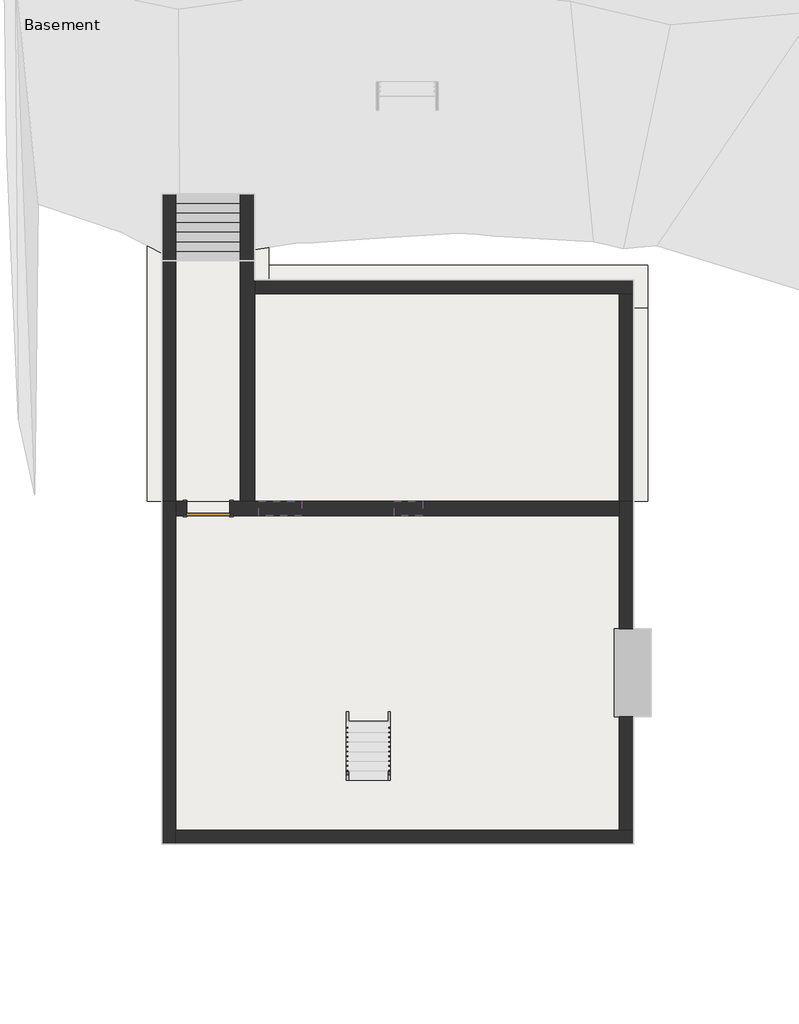
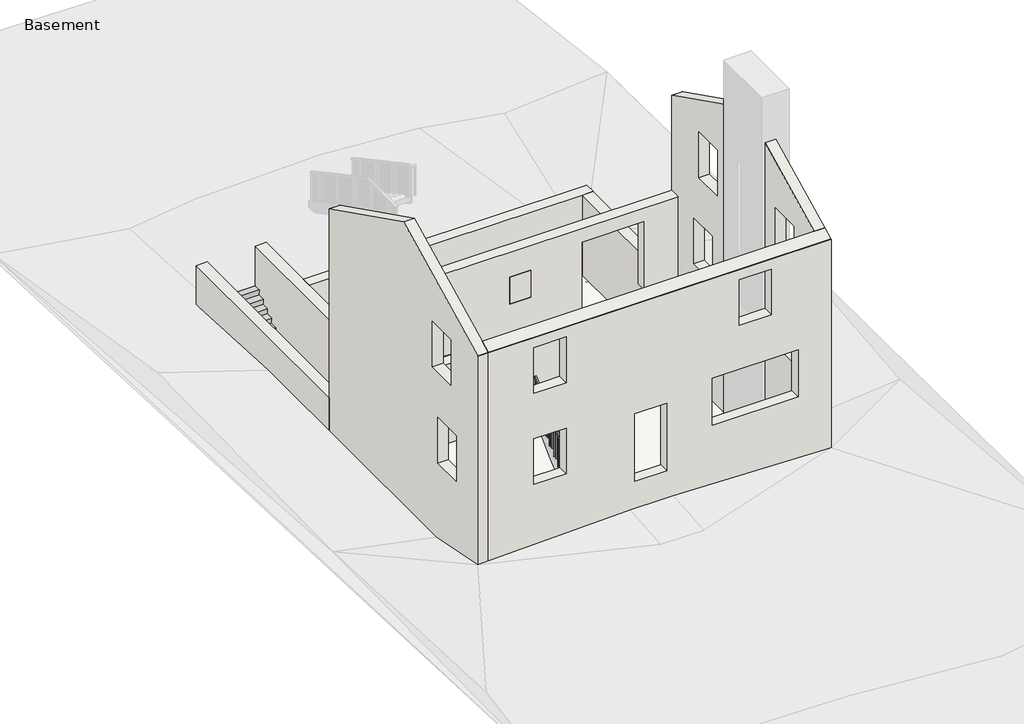
# One storey, part 1 of 2: 11 walls, 4 footings, 4 slabs, 2 railings, 1 door, 1 stair flight.
"""IFC4 building model written with IfcOpenShell, lengths in millimetres."""

import ifcopenshell
import ifcopenshell.guid

model = None  # the IFC model being written
_history = None  # IfcOwnerHistory: only IFC2X3 demands one
_inside = {}  # id of a spatial element -> (the spatial element, [elements in it])
_under = {}  # id of a project, library or spatial element -> (it, [spatial elements below it])
_declared = {}  # id of a project -> (the project, [libraries it declares])
_typed = {}  # id of a type object -> (the type object, [elements of that type])
_made_of = {}  # id of a material, layer set ... -> (it, [elements and type objects made of it])


def new_model(schema):
    """Start an empty IFC model of exactly this schema.

    Asked for "IFC4X3", IfcOpenShell would pick the latest addendum, in which some entities
    have other attributes; the version numbers below select the first issue.
    IFC2X3 requires an IfcOwnerHistory on every rooted entity: one is made here for all.
    """
    global model, _history
    if schema == "IFC4X3":
        model = ifcopenshell.file(schema_version=(4, 3, 0, 0))
    else:
        model = ifcopenshell.file(schema=schema)
    _inside.clear()
    _under.clear()
    _declared.clear()
    _typed.clear()
    _made_of.clear()
    _history = None
    if model.schema == "IFC2X3":
        org = make("IfcOrganization", Name="unknown")
        user = make(
            "IfcPersonAndOrganization",
            ThePerson=make("IfcPerson", FamilyName="unknown"),
            TheOrganization=org,
        )
        app = make(
            "IfcApplication",
            ApplicationDeveloper=org,
            Version="unknown",
            ApplicationFullName="unknown",
            ApplicationIdentifier="unknown",
        )
        _history = make(
            "IfcOwnerHistory",
            OwningUser=user,
            OwningApplication=app,
            ChangeAction="ADDED",
            CreationDate=0,
        )
    return model


def make(cls, **values):
    """One entity of the class cls with the attributes given. An attribute that is None is left unset."""
    return model.create_entity(
        cls, **{name: value for name, value in values.items() if value is not None}
    )


def rooted(cls, **values):
    """An entity with a GlobalId (a new one), such as an element, a storey or a relation."""
    return make(cls, GlobalId=ifcopenshell.guid.new(), OwnerHistory=_history, **values)


def si_unit(unit_type, name, prefix=None):
    """IfcSIUnit, for example si_unit("LENGTHUNIT", "METRE", prefix="MILLI")."""
    return make("IfcSIUnit", UnitType=unit_type, Prefix=prefix, Name=name)


def assignment(units):
    """IfcUnitAssignment: the units of a project."""
    return None if units is None else make("IfcUnitAssignment", Units=units)


def point(xyz):
    """IfcCartesianPoint."""
    return None if xyz is None else make("IfcCartesianPoint", Coordinates=xyz)


def direction(xyz):
    """IfcDirection."""
    return None if xyz is None else make("IfcDirection", DirectionRatios=xyz)


def frame(location, z_axis=None, x_axis=None):
    """IfcAxis2Placement3D, a coordinate frame: its origin and axes. An axis left out is left unset."""
    return make(
        "IfcAxis2Placement3D",
        Location=point(location),
        Axis=direction(z_axis),
        RefDirection=direction(x_axis),
    )


def origin():
    """The frame at (0, 0, 0) with its axes left unset."""
    return frame((0.0, 0.0, 0.0))


def origin_with_axes():
    """The frame at (0, 0, 0) with the z axis (0, 0, 1) and the x axis (1, 0, 0) written out."""
    return frame((0.0, 0.0, 0.0), z_axis=(0.0, 0.0, 1.0), x_axis=(1.0, 0.0, 0.0))


def place(relative_to, where):
    """IfcLocalPlacement: puts the frame where relative to a parent placement (None: the world)."""
    return make(
        "IfcLocalPlacement", PlacementRelTo=relative_to, RelativePlacement=where
    )


def context(
    kind, dimensions, precision=None, world=None, true_north=None, identifier=None
):
    """IfcGeometricRepresentationContext, for example the 3D "Model" context."""
    return make(
        "IfcGeometricRepresentationContext",
        ContextIdentifier=identifier,
        ContextType=kind,
        CoordinateSpaceDimension=dimensions,
        Precision=precision,
        WorldCoordinateSystem=world,
        TrueNorth=true_north,
    )


def project(units=None, contexts=None):
    """IfcProject with its units and contexts."""
    return rooted(
        "IfcProject",
        Name="project",
        RepresentationContexts=contexts,
        UnitsInContext=assignment(units),
    )


def spatial(cls, under=None, at=None, **own):
    """A site, building, storey or space (cls), placed at a placement, below another one or the project."""
    s = rooted(cls, ObjectPlacement=at, **own)
    if under is not None:
        _under.setdefault(under.id(), (under, []))[1].append(s)
    return s


def polyline(points):
    """IfcPolyline through the points."""
    return make("IfcPolyline", Points=[point(p) for p in points])


def outline(outer, holes=None, kind="AREA"):
    """IfcArbitraryClosedProfileDef: a profile drawn as a closed curve; with holes, ...WithVoids."""
    if holes is None:
        return make("IfcArbitraryClosedProfileDef", ProfileType=kind, OuterCurve=outer)
    return make(
        "IfcArbitraryProfileDefWithVoids",
        ProfileType=kind,
        OuterCurve=outer,
        InnerCurves=holes,
    )


def extrude(swept, where, along, depth):
    """IfcExtrudedAreaSolid: the profile swept, set in the frame where, extruded along a direction by depth."""
    return make(
        "IfcExtrudedAreaSolid",
        SweptArea=swept,
        Position=where,
        ExtrudedDirection=direction(along),
        Depth=depth,
    )


def faces_of(points, faces, orient=None, outer=None):
    """IfcFace entities. A face is a list of loops; a loop is a list of indices into points, from 0.

    orient and outer hold one flag for each loop. By default every Orientation is true, the
    first loop of a face is its IfcFaceOuterBound and the others are IfcFaceBound.
    """
    made = []
    for i, loops in enumerate(faces):
        bounds = []
        for j, loop in enumerate(loops):
            is_outer = j == 0 if outer is None else outer[i][j]
            bounds.append(
                make(
                    "IfcFaceOuterBound" if is_outer else "IfcFaceBound",
                    Bound=make("IfcPolyLoop", Polygon=[points[k] for k in loop]),
                    Orientation=True if orient is None else orient[i][j],
                )
            )
        made.append(make("IfcFace", Bounds=bounds))
    return made


def faceted_brep(points, faces, orient=None, outer=None, voids=None):
    """IfcFacetedBrep: a solid bounded by flat faces; with voids (closed shells), ...WithVoids."""
    shared = [point(p) for p in points]
    hull = make("IfcClosedShell", CfsFaces=faces_of(shared, faces, orient, outer))
    if voids is None:
        return make("IfcFacetedBrep", Outer=hull)
    return make(
        "IfcFacetedBrepWithVoids",
        Outer=hull,
        Voids=[
            make(cls, CfsFaces=faces_of(shared, fs, o, b)) for cls, fs, o, b in voids
        ],
    )


def shape(context_of_items, identifier, shape_type, items):
    """IfcShapeRepresentation: the items that make up one representation, for example the "Body"."""
    return make(
        "IfcShapeRepresentation",
        ContextOfItems=context_of_items,
        RepresentationIdentifier=identifier,
        RepresentationType=shape_type,
        Items=items,
    )


def source(mapping_origin, context_of_items, identifier, shape_type, items):
    """IfcRepresentationMap: a shape defined once, which mapped items show again and again."""
    return make(
        "IfcRepresentationMap",
        MappingOrigin=mapping_origin,
        MappedRepresentation=shape(context_of_items, identifier, shape_type, items),
    )


def transform(
    local_origin,
    x_axis=None,
    y_axis=None,
    z_axis=None,
    scale=None,
    scale2=None,
    scale3=None,
    uniform=True,
):
    """IfcCartesianTransformationOperator3D, or its non-uniform kind. x_axis, y_axis, z_axis: its Axis1, 2, 3."""
    if uniform:
        return make(
            "IfcCartesianTransformationOperator3D",
            Axis1=direction(x_axis),
            Axis2=direction(y_axis),
            LocalOrigin=point(local_origin),
            Scale=scale,
            Axis3=direction(z_axis),
        )
    return make(
        "IfcCartesianTransformationOperator3DnonUniform",
        Axis1=direction(x_axis),
        Axis2=direction(y_axis),
        LocalOrigin=point(local_origin),
        Scale=scale,
        Axis3=direction(z_axis),
        Scale2=scale2,
        Scale3=scale3,
    )


def mapped(mapping_source, mapping_target):
    """IfcMappedItem: shows the shape of a source again, moved by a transform."""
    return make(
        "IfcMappedItem", MappingSource=mapping_source, MappingTarget=mapping_target
    )


def made_of(thing, what):
    """Note that an element or type object is made of a material, layer set ...; save() writes the relation."""
    if what is not None:
        _made_of.setdefault(what.id(), (what, []))[1].append(thing)
    return thing


def element(
    cls,
    number,
    at=None,
    inside=None,
    cuts=None,
    type_object=None,
    material=None,
    context=None,
    identifier="Body",
    shape_type=None,
    held_by="IfcProductDefinitionShape",
    body=None,
    shapes=None,
    **own,
):
    """One element of the class cls, such as IfcWall. Its Tag is "e" and its number.

    at: its placement. inside: the storey or other place that contains it. cuts: it is an
    opening in that element (IfcRelVoidsElement). A single representation is given by context,
    identifier, shape_type and body (its items); several are given by shapes. held_by: the class
    of the entity that holds the representations. save() writes the other relations.
    """
    e = rooted(cls, Tag="e%d" % number, ObjectPlacement=at, **own)
    if body is not None:
        shapes = [shape(context, identifier, shape_type, body)]
    if shapes is not None:
        e.Representation = make(held_by, Representations=shapes)
    if inside is not None:
        _inside.setdefault(inside.id(), (inside, []))[1].append(e)
    if cuts is not None:
        rooted(
            "IfcRelVoidsElement", RelatingBuildingElement=cuts, RelatedOpeningElement=e
        )
    if type_object is not None:
        _typed.setdefault(type_object.id(), (type_object, []))[1].append(e)
    return made_of(e, material)


def aggregate(whole, parts):
    """IfcRelAggregates: a whole, such as a stair, and the parts it consists of."""
    return rooted("IfcRelAggregates", RelatingObject=whole, RelatedObjects=parts)


def save(model, path):
    """Write the relations noted so far, then the file.

    IfcRelAggregates (storeys below a building ...), IfcRelContainedInSpatialStructure (elements
    in a storey), IfcRelDefinesByType, IfcRelAssociatesMaterial and IfcRelDeclares: one each for
    every whole, place, type object, material and project.
    """
    for whole, parts in _under.values():
        aggregate(whole, parts)
    for where, things in _inside.values():
        rooted(
            "IfcRelContainedInSpatialStructure",
            RelatedElements=things,
            RelatingStructure=where,
        )
    for kind, things in _typed.values():
        rooted("IfcRelDefinesByType", RelatedObjects=things, RelatingType=kind)
    for what, things in _made_of.values():
        rooted("IfcRelAssociatesMaterial", RelatedObjects=things, RelatingMaterial=what)
    for by, libraries in _declared.values():
        rooted("IfcRelDeclares", RelatingContext=by, RelatedDefinitions=libraries)
    model.write(path)


def door_03272193(model_context):
    return source(origin(), model_context, "Body", "SweptSolid", [
        extrude(outline(polyline([(2209.8, -533.4), (0.0, -533.4), (0.0, -457.2), (2133.6, -457.2), (2133.6, 457.2), (0.0, 457.2), (0.0, 533.4), (2209.8, 533.4), (2209.8, -533.4)])), frame((0.0, 152.4, 0.0), z_axis=(0.0, 1.0, 0.0), x_axis=(0.0, 0.0, 1.0)), (0.0, 0.0, 1.0), 25.4),
        extrude(outline(polyline([(2209.8, 533.4), (2209.8, -533.4), (0.0, -533.4), (0.0, -457.2), (2133.6, -457.2), (2133.6, 457.2), (0.0, 457.2), (0.0, 533.4), (2209.8, 533.4)])), frame((0.0, -177.8, 0.0), z_axis=(0.0, 1.0, 0.0), x_axis=(0.0, 0.0, 1.0)), (0.0, 0.0, 1.0), 25.4),
        extrude(outline(polyline([(457.2, 101.6), (-457.2, 101.6), (-457.2, 152.4), (457.2, 152.4), (457.2, 101.6)])), origin_with_axes(), (0.0, 0.0, 1.0), 2133.6),
    ])


model = new_model("IFC4")

# Units and contexts
model_context = context("Model", 3, world=origin())
ifc_project = project(units=[si_unit("LENGTHUNIT", "METRE", prefix="MILLI")], contexts=[model_context])

# Site, building, storey
site = spatial("IfcSite", under=ifc_project)
building = spatial("IfcBuilding", under=site)
storey = spatial("IfcBuildingStorey", under=building, Name="Basement", Elevation=-2667.0)

# Door
placement = place(None, origin())
door_shape = door_03272193(model_context)
element("IfcDoor", 1, ObjectType="Single-Flush : 36\" x 84\"", at=placement, inside=storey, context=model_context, shape_type="MappedRepresentation", body=[
    mapped(door_shape, transform((-4998.5803068, 2999.6888758, -2667.0), x_axis=(-1.0, 0.0, 0.0), y_axis=(0.0, -1.0, 0.0), z_axis=(0.0, 0.0, 1.0))),
])

# Footings
element("IfcFooting", 2, ObjectType="Bearing Footing - 36\" x 12\"", at=placement, inside=storey, context=model_context, shape_type="SweptSolid", body=[
    extrude(outline(polyline([(-5379.5803068, 3152.0888758), (-6293.9803068, 3152.0888758), (-6293.9803068, 10010.0888758), (-5379.5803068, 10010.0888758), (-5379.5803068, 3152.0888758)])), frame((0.0, 0.0, -3073.4), z_axis=(0.0, 0.0, 1.0), x_axis=(1.0, 0.0, 0.0)), (0.0, 0.0, 1.0), 304.8),
])
element("IfcFooting", 3, ObjectType="Bearing Footing - 36\" x 12\"", at=placement, inside=storey, context=model_context, shape_type="Brep", body=[
    faceted_brep([(-3703.1803068, 7266.8888758, -2768.6), (3459.6196932, 7266.8888758, -2768.6), (4374.0196932, 7266.8888758, -2768.6), (4374.0196932, 8181.2888758, -2768.6), (-3703.1803068, 8181.2888758, -2768.6), (-3703.1803068, 8181.2888758, -3073.4), (4374.0196932, 8181.2888758, -3073.4), (-3703.1803068, 7266.8888758, -3073.4), (4374.0196932, 7266.8888758, -3073.4), (3459.6196932, 7266.8888758, -3073.4)], [[[0, 1, 2, 3, 4]], [[5, 4, 3, 6]], [[7, 5, 6, 8, 9]], [[0, 7, 9, 8, 2, 1]], [[0, 4, 5, 7]], [[3, 2, 8, 6]]]),
])
element("IfcFooting", 4, ObjectType="Bearing Footing - 36\" x 12\"", at=placement, inside=storey, context=model_context, shape_type="SweptSolid", body=[
    extrude(outline(polyline([(4374.0196932, 3152.0888758), (3459.6196932, 3152.0888758), (3459.6196932, 7266.8888758), (4374.0196932, 7266.8888758), (4374.0196932, 3152.0888758)])), frame((0.0, 0.0, -3073.4), z_axis=(0.0, 0.0, 1.0), x_axis=(1.0, 0.0, 0.0)), (0.0, 0.0, 1.0), 304.8),
])
element("IfcFooting", 5, ObjectType="Bearing Footing - 36\" x 12\"", at=placement, inside=storey, context=model_context, shape_type="Brep", body=[
    faceted_brep([(-3703.1803068, 3152.0888758, -2768.6), (-4617.5803068, 3152.0888758, -2768.6), (-4617.5803068, 3152.0888758, -3073.4), (-3703.1803068, 3152.0888758, -3073.4), (-4617.5803068, 10010.0888758, -2768.6), (-3703.1803068, 10010.0888758, -2768.6), (-3703.1803068, 10010.0888758, -3073.4), (-4617.5803068, 10010.0888758, -3073.4), (-3703.1803068, 7266.8888758, -2768.6), (-3703.1803068, 8181.2888758, -2768.6), (-3703.1803068, 8181.2888758, -3073.4), (-3703.1803068, 7266.8888758, -3073.4)], [[[0, 1, 2, 3]], [[4, 5, 6, 7]], [[0, 8, 9, 5, 4, 1]], [[2, 1, 4, 7]], [[3, 2, 7, 6, 10, 11]], [[0, 3, 11, 10, 6, 5, 9, 8]]]),
])

# Railings
element("IfcRailing", 6, ObjectType="Handrail - Rectangular", at=placement, inside=storey, context=model_context, shape_type="SweptSolid", body=[
    extrude(outline(polyline([(-2791.5111242, -1631.7331862), (-2791.5111242, -1562.1), (-149.9111242, 914.4), (-149.9111242, 844.7668138), (-2791.5111242, -1631.7331862)])), frame((-1163.1803068, 0.0, 0.0), z_axis=(1.0, 0.0, 0.0), x_axis=(0.0, 1.0, 0.0)), (0.0, 0.0, 1.0), 50.8),
    extrude(outline(polyline([(-261.0361242, 740.5871263), (-241.9861242, 758.4465013), (-241.9861242, -190.5), (-261.0361242, -190.5), (-261.0361242, 740.5871263)])), frame((-1147.3053068, 0.0, 0.0), z_axis=(1.0, 0.0, 0.0), x_axis=(0.0, 1.0, 0.0)), (0.0, 0.0, 1.0), 19.05),
    extrude(outline(polyline([(-362.6361242, 645.3371263), (-343.5861242, 663.1965013), (-343.5861242, -190.5), (-362.6361242, -190.5), (-362.6361242, 645.3371263)])), frame((-1147.3053068, 0.0, 0.0), z_axis=(1.0, 0.0, 0.0), x_axis=(0.0, 1.0, 0.0)), (0.0, 0.0, 1.0), 19.05),
    extrude(outline(polyline([(-464.2361242, 550.0871263), (-445.1861242, 567.9465013), (-445.1861242, -381.0), (-464.2361242, -381.0), (-464.2361242, 550.0871263)])), frame((-1147.3053068, 0.0, 0.0), z_axis=(1.0, 0.0, 0.0), x_axis=(0.0, 1.0, 0.0)), (0.0, 0.0, 1.0), 19.05),
    extrude(outline(polyline([(-565.8361242, 454.8371263), (-546.7861242, 472.6965013), (-546.7861242, -381.0), (-565.8361242, -381.0), (-565.8361242, 454.8371263)])), frame((-1147.3053068, 0.0, 0.0), z_axis=(1.0, 0.0, 0.0), x_axis=(0.0, 1.0, 0.0)), (0.0, 0.0, 1.0), 19.05),
    extrude(outline(polyline([(-667.4361242, 359.5871263), (-648.3861242, 377.4465013), (-648.3861242, -571.5), (-667.4361242, -571.5), (-667.4361242, 359.5871263)])), frame((-1147.3053068, 0.0, 0.0), z_axis=(1.0, 0.0, 0.0), x_axis=(0.0, 1.0, 0.0)), (0.0, 0.0, 1.0), 19.05),
    extrude(outline(polyline([(-769.0361242, 264.3371263), (-749.9861242, 282.1965013), (-749.9861242, -571.5), (-769.0361242, -571.5), (-769.0361242, 264.3371263)])), frame((-1147.3053068, 0.0, 0.0), z_axis=(1.0, 0.0, 0.0), x_axis=(0.0, 1.0, 0.0)), (0.0, 0.0, 1.0), 19.05),
    extrude(outline(polyline([(-870.6361242, 169.0871263), (-851.5861242, 186.9465013), (-851.5861242, -762.0), (-870.6361242, -762.0), (-870.6361242, 169.0871263)])), frame((-1147.3053068, 0.0, 0.0), z_axis=(1.0, 0.0, 0.0), x_axis=(0.0, 1.0, 0.0)), (0.0, 0.0, 1.0), 19.05),
    extrude(outline(polyline([(-972.2361242, 73.8371263), (-953.1861242, 91.6965013), (-953.1861242, -762.0), (-972.2361242, -762.0), (-972.2361242, 73.8371263)])), frame((-1147.3053068, 0.0, 0.0), z_axis=(1.0, 0.0, 0.0), x_axis=(0.0, 1.0, 0.0)), (0.0, 0.0, 1.0), 19.05),
    extrude(outline(polyline([(-1073.8361242, -21.4128737), (-1054.7861242, -3.5534987), (-1054.7861242, -952.5), (-1073.8361242, -952.5), (-1073.8361242, -21.4128737)])), frame((-1147.3053068, 0.0, 0.0), z_axis=(1.0, 0.0, 0.0), x_axis=(0.0, 1.0, 0.0)), (0.0, 0.0, 1.0), 19.05),
    extrude(outline(polyline([(-1175.4361242, -116.6628737), (-1156.3861242, -98.8034987), (-1156.3861242, -952.5), (-1175.4361242, -952.5), (-1175.4361242, -116.6628737)])), frame((-1147.3053068, 0.0, 0.0), z_axis=(1.0, 0.0, 0.0), x_axis=(0.0, 1.0, 0.0)), (0.0, 0.0, 1.0), 19.05),
    extrude(outline(polyline([(-1277.0361242, -211.9128737), (-1257.9861242, -194.0534987), (-1257.9861242, -1143.0), (-1277.0361242, -1143.0), (-1277.0361242, -211.9128737)])), frame((-1147.3053068, 0.0, 0.0), z_axis=(1.0, 0.0, 0.0), x_axis=(0.0, 1.0, 0.0)), (0.0, 0.0, 1.0), 19.05),
    extrude(outline(polyline([(-1378.6361242, -307.1628737), (-1359.5861242, -289.3034987), (-1359.5861242, -1143.0), (-1378.6361242, -1143.0), (-1378.6361242, -307.1628737)])), frame((-1147.3053068, 0.0, 0.0), z_axis=(1.0, 0.0, 0.0), x_axis=(0.0, 1.0, 0.0)), (0.0, 0.0, 1.0), 19.05),
    extrude(outline(polyline([(-1480.2361242, -402.4128737), (-1461.1861242, -384.5534987), (-1461.1861242, -1333.5), (-1480.2361242, -1333.5), (-1480.2361242, -402.4128737)])), frame((-1147.3053068, 0.0, 0.0), z_axis=(1.0, 0.0, 0.0), x_axis=(0.0, 1.0, 0.0)), (0.0, 0.0, 1.0), 19.05),
    extrude(outline(polyline([(-1581.8361242, -497.6628737), (-1562.7861242, -479.8034987), (-1562.7861242, -1333.5), (-1581.8361242, -1333.5), (-1581.8361242, -497.6628737)])), frame((-1147.3053068, 0.0, 0.0), z_axis=(1.0, 0.0, 0.0), x_axis=(0.0, 1.0, 0.0)), (0.0, 0.0, 1.0), 19.05),
    extrude(outline(polyline([(-1683.4361242, -592.9128737), (-1664.3861242, -575.0534987), (-1664.3861242, -1524.0), (-1683.4361242, -1524.0), (-1683.4361242, -592.9128737)])), frame((-1147.3053068, 0.0, 0.0), z_axis=(1.0, 0.0, 0.0), x_axis=(0.0, 1.0, 0.0)), (0.0, 0.0, 1.0), 19.05),
    extrude(outline(polyline([(-1785.0361242, -688.1628737), (-1765.9861242, -670.3034987), (-1765.9861242, -1524.0), (-1785.0361242, -1524.0), (-1785.0361242, -688.1628737)])), frame((-1147.3053068, 0.0, 0.0), z_axis=(1.0, 0.0, 0.0), x_axis=(0.0, 1.0, 0.0)), (0.0, 0.0, 1.0), 19.05),
    extrude(outline(polyline([(-1886.6361242, -783.4128737), (-1867.5861242, -765.5534987), (-1867.5861242, -1714.5), (-1886.6361242, -1714.5), (-1886.6361242, -783.4128737)])), frame((-1147.3053068, 0.0, 0.0), z_axis=(1.0, 0.0, 0.0), x_axis=(0.0, 1.0, 0.0)), (0.0, 0.0, 1.0), 19.05),
    extrude(outline(polyline([(-1988.2361242, -878.6628737), (-1969.1861242, -860.8034987), (-1969.1861242, -1714.5), (-1988.2361242, -1714.5), (-1988.2361242, -878.6628737)])), frame((-1147.3053068, 0.0, 0.0), z_axis=(1.0, 0.0, 0.0), x_axis=(0.0, 1.0, 0.0)), (0.0, 0.0, 1.0), 19.05),
    extrude(outline(polyline([(-2089.8361242, -973.9128737), (-2070.7861242, -956.0534987), (-2070.7861242, -1905.0), (-2089.8361242, -1905.0), (-2089.8361242, -973.9128737)])), frame((-1147.3053068, 0.0, 0.0), z_axis=(1.0, 0.0, 0.0), x_axis=(0.0, 1.0, 0.0)), (0.0, 0.0, 1.0), 19.05),
    extrude(outline(polyline([(-2191.4361242, -1069.1628737), (-2172.3861242, -1051.3034987), (-2172.3861242, -1905.0), (-2191.4361242, -1905.0), (-2191.4361242, -1069.1628737)])), frame((-1147.3053068, 0.0, 0.0), z_axis=(1.0, 0.0, 0.0), x_axis=(0.0, 1.0, 0.0)), (0.0, 0.0, 1.0), 19.05),
    extrude(outline(polyline([(-2293.0361242, -1164.4128737), (-2273.9861242, -1146.5534987), (-2273.9861242, -2095.5), (-2293.0361242, -2095.5), (-2293.0361242, -1164.4128737)])), frame((-1147.3053068, 0.0, 0.0), z_axis=(1.0, 0.0, 0.0), x_axis=(0.0, 1.0, 0.0)), (0.0, 0.0, 1.0), 19.05),
    extrude(outline(polyline([(-2394.6361242, -1259.6628737), (-2375.5861242, -1241.8034987), (-2375.5861242, -2095.5), (-2394.6361242, -2095.5), (-2394.6361242, -1259.6628737)])), frame((-1147.3053068, 0.0, 0.0), z_axis=(1.0, 0.0, 0.0), x_axis=(0.0, 1.0, 0.0)), (0.0, 0.0, 1.0), 19.05),
    extrude(outline(polyline([(-2496.2361242, -1354.9128737), (-2477.1861242, -1337.0534987), (-2477.1861242, -2286.0), (-2496.2361242, -2286.0), (-2496.2361242, -1354.9128737)])), frame((-1147.3053068, 0.0, 0.0), z_axis=(1.0, 0.0, 0.0), x_axis=(0.0, 1.0, 0.0)), (0.0, 0.0, 1.0), 19.05),
    extrude(outline(polyline([(-2597.8361242, -1450.1628737), (-2578.7861242, -1432.3034987), (-2578.7861242, -2286.0), (-2597.8361242, -2286.0), (-2597.8361242, -1450.1628737)])), frame((-1147.3053068, 0.0, 0.0), z_axis=(1.0, 0.0, 0.0), x_axis=(0.0, 1.0, 0.0)), (0.0, 0.0, 1.0), 19.05),
    extrude(outline(polyline([(-2699.4361242, -1545.4128737), (-2680.3861242, -1527.5534987), (-2680.3861242, -2476.5), (-2699.4361242, -2476.5), (-2699.4361242, -1545.4128737)])), frame((-1147.3053068, 0.0, 0.0), z_axis=(1.0, 0.0, 0.0), x_axis=(0.0, 1.0, 0.0)), (0.0, 0.0, 1.0), 19.05),
    extrude(outline(polyline([(-168.9611242, 826.9074388), (-149.9111242, 844.7668138), (-149.9111242, -190.5), (-168.9611242, -190.5), (-168.9611242, 826.9074388)])), frame((-1147.3053068, 0.0, 0.0), z_axis=(1.0, 0.0, 0.0), x_axis=(0.0, 1.0, 0.0)), (0.0, 0.0, 1.0), 19.05),
    extrude(outline(polyline([(-2791.5111242, -1631.7331862), (-2772.4611242, -1613.8738112), (-2772.4611242, -2476.5), (-2791.5111242, -2476.5), (-2791.5111242, -1631.7331862)])), frame((-1147.3053068, 0.0, 0.0), z_axis=(1.0, 0.0, 0.0), x_axis=(0.0, 1.0, 0.0)), (0.0, 0.0, 1.0), 19.05),
])
element("IfcRailing", 7, ObjectType="Handrail - Rectangular", at=placement, inside=storey, context=model_context, shape_type="SweptSolid", body=[
    extrude(outline(polyline([(-2791.5111242, -1631.7331862), (-2791.5111242, -1562.1), (-149.9111242, 914.4), (-149.9111242, 844.7668138), (-2791.5111242, -1631.7331862)])), frame((-2052.1803068, 0.0, 0.0), z_axis=(1.0, 0.0, 0.0), x_axis=(0.0, 1.0, 0.0)), (0.0, 0.0, 1.0), 50.8),
    extrude(outline(polyline([(-241.9861242, 758.4465013), (-241.9861242, -190.5), (-261.0361242, -190.5), (-261.0361242, 740.5871263), (-241.9861242, 758.4465013)])), frame((-2036.3053068, 0.0, 0.0), z_axis=(1.0, 0.0, 0.0), x_axis=(0.0, 1.0, 0.0)), (0.0, 0.0, 1.0), 19.05),
    extrude(outline(polyline([(-343.5861242, 663.1965013), (-343.5861242, -190.5), (-362.6361242, -190.5), (-362.6361242, 645.3371263), (-343.5861242, 663.1965013)])), frame((-2036.3053068, 0.0, 0.0), z_axis=(1.0, 0.0, 0.0), x_axis=(0.0, 1.0, 0.0)), (0.0, 0.0, 1.0), 19.05),
    extrude(outline(polyline([(-445.1861242, 567.9465013), (-445.1861242, -381.0), (-464.2361242, -381.0), (-464.2361242, 550.0871263), (-445.1861242, 567.9465013)])), frame((-2036.3053068, 0.0, 0.0), z_axis=(1.0, 0.0, 0.0), x_axis=(0.0, 1.0, 0.0)), (0.0, 0.0, 1.0), 19.05),
    extrude(outline(polyline([(-546.7861242, 472.6965013), (-546.7861242, -381.0), (-565.8361242, -381.0), (-565.8361242, 454.8371263), (-546.7861242, 472.6965013)])), frame((-2036.3053068, 0.0, 0.0), z_axis=(1.0, 0.0, 0.0), x_axis=(0.0, 1.0, 0.0)), (0.0, 0.0, 1.0), 19.05),
    extrude(outline(polyline([(-648.3861242, 377.4465013), (-648.3861242, -571.5), (-667.4361242, -571.5), (-667.4361242, 359.5871263), (-648.3861242, 377.4465013)])), frame((-2036.3053068, 0.0, 0.0), z_axis=(1.0, 0.0, 0.0), x_axis=(0.0, 1.0, 0.0)), (0.0, 0.0, 1.0), 19.05),
    extrude(outline(polyline([(-749.9861242, 282.1965013), (-749.9861242, -571.5), (-769.0361242, -571.5), (-769.0361242, 264.3371263), (-749.9861242, 282.1965013)])), frame((-2036.3053068, 0.0, 0.0), z_axis=(1.0, 0.0, 0.0), x_axis=(0.0, 1.0, 0.0)), (0.0, 0.0, 1.0), 19.05),
    extrude(outline(polyline([(-851.5861242, 186.9465013), (-851.5861242, -762.0), (-870.6361242, -762.0), (-870.6361242, 169.0871263), (-851.5861242, 186.9465013)])), frame((-2036.3053068, 0.0, 0.0), z_axis=(1.0, 0.0, 0.0), x_axis=(0.0, 1.0, 0.0)), (0.0, 0.0, 1.0), 19.05),
    extrude(outline(polyline([(-953.1861242, 91.6965013), (-953.1861242, -762.0), (-972.2361242, -762.0), (-972.2361242, 73.8371263), (-953.1861242, 91.6965013)])), frame((-2036.3053068, 0.0, 0.0), z_axis=(1.0, 0.0, 0.0), x_axis=(0.0, 1.0, 0.0)), (0.0, 0.0, 1.0), 19.05),
    extrude(outline(polyline([(-1054.7861242, -3.5534987), (-1054.7861242, -952.5), (-1073.8361242, -952.5), (-1073.8361242, -21.4128737), (-1054.7861242, -3.5534987)])), frame((-2036.3053068, 0.0, 0.0), z_axis=(1.0, 0.0, 0.0), x_axis=(0.0, 1.0, 0.0)), (0.0, 0.0, 1.0), 19.05),
    extrude(outline(polyline([(-1156.3861242, -98.8034987), (-1156.3861242, -952.5), (-1175.4361242, -952.5), (-1175.4361242, -116.6628737), (-1156.3861242, -98.8034987)])), frame((-2036.3053068, 0.0, 0.0), z_axis=(1.0, 0.0, 0.0), x_axis=(0.0, 1.0, 0.0)), (0.0, 0.0, 1.0), 19.05),
    extrude(outline(polyline([(-1257.9861242, -194.0534987), (-1257.9861242, -1143.0), (-1277.0361242, -1143.0), (-1277.0361242, -211.9128737), (-1257.9861242, -194.0534987)])), frame((-2036.3053068, 0.0, 0.0), z_axis=(1.0, 0.0, 0.0), x_axis=(0.0, 1.0, 0.0)), (0.0, 0.0, 1.0), 19.05),
    extrude(outline(polyline([(-1359.5861242, -289.3034987), (-1359.5861242, -1143.0), (-1378.6361242, -1143.0), (-1378.6361242, -307.1628737), (-1359.5861242, -289.3034987)])), frame((-2036.3053068, 0.0, 0.0), z_axis=(1.0, 0.0, 0.0), x_axis=(0.0, 1.0, 0.0)), (0.0, 0.0, 1.0), 19.05),
    extrude(outline(polyline([(-1461.1861242, -384.5534987), (-1461.1861242, -1333.5), (-1480.2361242, -1333.5), (-1480.2361242, -402.4128737), (-1461.1861242, -384.5534987)])), frame((-2036.3053068, 0.0, 0.0), z_axis=(1.0, 0.0, 0.0), x_axis=(0.0, 1.0, 0.0)), (0.0, 0.0, 1.0), 19.05),
    extrude(outline(polyline([(-1562.7861242, -479.8034987), (-1562.7861242, -1333.5), (-1581.8361242, -1333.5), (-1581.8361242, -497.6628737), (-1562.7861242, -479.8034987)])), frame((-2036.3053068, 0.0, 0.0), z_axis=(1.0, 0.0, 0.0), x_axis=(0.0, 1.0, 0.0)), (0.0, 0.0, 1.0), 19.05),
    extrude(outline(polyline([(-1664.3861242, -575.0534987), (-1664.3861242, -1524.0), (-1683.4361242, -1524.0), (-1683.4361242, -592.9128737), (-1664.3861242, -575.0534987)])), frame((-2036.3053068, 0.0, 0.0), z_axis=(1.0, 0.0, 0.0), x_axis=(0.0, 1.0, 0.0)), (0.0, 0.0, 1.0), 19.05),
    extrude(outline(polyline([(-1765.9861242, -670.3034987), (-1765.9861242, -1524.0), (-1785.0361242, -1524.0), (-1785.0361242, -688.1628737), (-1765.9861242, -670.3034987)])), frame((-2036.3053068, 0.0, 0.0), z_axis=(1.0, 0.0, 0.0), x_axis=(0.0, 1.0, 0.0)), (0.0, 0.0, 1.0), 19.05),
    extrude(outline(polyline([(-1867.5861242, -765.5534987), (-1867.5861242, -1714.5), (-1886.6361242, -1714.5), (-1886.6361242, -783.4128737), (-1867.5861242, -765.5534987)])), frame((-2036.3053068, 0.0, 0.0), z_axis=(1.0, 0.0, 0.0), x_axis=(0.0, 1.0, 0.0)), (0.0, 0.0, 1.0), 19.05),
    extrude(outline(polyline([(-1969.1861242, -860.8034987), (-1969.1861242, -1714.5), (-1988.2361242, -1714.5), (-1988.2361242, -878.6628737), (-1969.1861242, -860.8034987)])), frame((-2036.3053068, 0.0, 0.0), z_axis=(1.0, 0.0, 0.0), x_axis=(0.0, 1.0, 0.0)), (0.0, 0.0, 1.0), 19.05),
    extrude(outline(polyline([(-2070.7861242, -956.0534987), (-2070.7861242, -1905.0), (-2089.8361242, -1905.0), (-2089.8361242, -973.9128737), (-2070.7861242, -956.0534987)])), frame((-2036.3053068, 0.0, 0.0), z_axis=(1.0, 0.0, 0.0), x_axis=(0.0, 1.0, 0.0)), (0.0, 0.0, 1.0), 19.05),
    extrude(outline(polyline([(-2172.3861242, -1051.3034987), (-2172.3861242, -1905.0), (-2191.4361242, -1905.0), (-2191.4361242, -1069.1628737), (-2172.3861242, -1051.3034987)])), frame((-2036.3053068, 0.0, 0.0), z_axis=(1.0, 0.0, 0.0), x_axis=(0.0, 1.0, 0.0)), (0.0, 0.0, 1.0), 19.05),
    extrude(outline(polyline([(-2273.9861242, -1146.5534987), (-2273.9861242, -2095.5), (-2293.0361242, -2095.5), (-2293.0361242, -1164.4128737), (-2273.9861242, -1146.5534987)])), frame((-2036.3053068, 0.0, 0.0), z_axis=(1.0, 0.0, 0.0), x_axis=(0.0, 1.0, 0.0)), (0.0, 0.0, 1.0), 19.05),
    extrude(outline(polyline([(-2375.5861242, -1241.8034987), (-2375.5861242, -2095.5), (-2394.6361242, -2095.5), (-2394.6361242, -1259.6628737), (-2375.5861242, -1241.8034987)])), frame((-2036.3053068, 0.0, 0.0), z_axis=(1.0, 0.0, 0.0), x_axis=(0.0, 1.0, 0.0)), (0.0, 0.0, 1.0), 19.05),
    extrude(outline(polyline([(-2477.1861242, -1337.0534987), (-2477.1861242, -2286.0), (-2496.2361242, -2286.0), (-2496.2361242, -1354.9128737), (-2477.1861242, -1337.0534987)])), frame((-2036.3053068, 0.0, 0.0), z_axis=(1.0, 0.0, 0.0), x_axis=(0.0, 1.0, 0.0)), (0.0, 0.0, 1.0), 19.05),
    extrude(outline(polyline([(-2578.7861242, -1432.3034987), (-2578.7861242, -2286.0), (-2597.8361242, -2286.0), (-2597.8361242, -1450.1628737), (-2578.7861242, -1432.3034987)])), frame((-2036.3053068, 0.0, 0.0), z_axis=(1.0, 0.0, 0.0), x_axis=(0.0, 1.0, 0.0)), (0.0, 0.0, 1.0), 19.05),
    extrude(outline(polyline([(-2680.3861242, -1527.5534987), (-2680.3861242, -2476.5), (-2699.4361242, -2476.5), (-2699.4361242, -1545.4128737), (-2680.3861242, -1527.5534987)])), frame((-2036.3053068, 0.0, 0.0), z_axis=(1.0, 0.0, 0.0), x_axis=(0.0, 1.0, 0.0)), (0.0, 0.0, 1.0), 19.05),
    extrude(outline(polyline([(-149.9111242, 844.7668138), (-149.9111242, -190.5), (-168.9611242, -190.5), (-168.9611242, 826.9074388), (-149.9111242, 844.7668138)])), frame((-2036.3053068, 0.0, 0.0), z_axis=(1.0, 0.0, 0.0), x_axis=(0.0, 1.0, 0.0)), (0.0, 0.0, 1.0), 19.05),
    extrude(outline(polyline([(-2772.4611242, -1613.8738112), (-2772.4611242, -2476.5), (-2791.5111242, -2476.5), (-2791.5111242, -1631.7331862), (-2772.4611242, -1613.8738112)])), frame((-2036.3053068, 0.0, 0.0), z_axis=(1.0, 0.0, 0.0), x_axis=(0.0, 1.0, 0.0)), (0.0, 0.0, 1.0), 19.05),
])

# Slabs
element("IfcSlab", 8, ObjectType="4\" Concrete", at=placement, inside=storey, context=model_context, shape_type="SweptSolid", body=[
    extrude(outline(polyline([(-5684.3803068, 8384.4888758), (-4312.7803068, 8384.4888758), (-4312.7803068, 3152.0888758), (-5684.3803068, 3152.0888758), (-5684.3803068, 8384.4888758)])), frame((0.0, 0.0, -2768.6), z_axis=(0.0, 0.0, 1.0), x_axis=(1.0, 0.0, 0.0)), (0.0, 0.0, 1.0), 101.6),
])
element("IfcSlab", 9, ObjectType="Pad 1", at=placement, inside=storey, context=model_context, shape_type="SweptSolid", body=[
    extrude(outline(polyline([(4069.2196932, 434.2888758), (4450.2196932, 434.2888758), (4450.2196932, -1445.3111242), (4069.2196932, -1445.3111242), (4069.2196932, -4163.1111242), (-5989.1803068, -4163.1111242), (-5989.1803068, 3152.0888758), (4069.2196932, 3152.0888758), (4069.2196932, 434.2888758)])), frame((0.0, 0.0, -2774.95), z_axis=(0.0, 0.0, 1.0), x_axis=(1.0, 0.0, 0.0)), (0.0, 0.0, 1.0), 6.35),
])
element("IfcSlab", 10, ObjectType="Pad 1", at=placement, inside=storey, context=model_context, shape_type="SweptSolid", body=[
    extrude(outline(polyline([(-5989.1803068, 8275.4102719), (-4007.9803068, 8275.4102719), (-4007.9803068, 7876.4888758), (4069.2196932, 7876.4888758), (4069.2196932, 3152.0888758), (-5989.1803068, 3152.0888758), (-5989.1803068, 8275.4102719)])), frame((0.0, 0.0, -2774.95), z_axis=(0.0, 0.0, 1.0), x_axis=(1.0, 0.0, 0.0)), (0.0, 0.0, 1.0), 6.35),
])
element("IfcSlab", 11, ObjectType="Pad 1", at=placement, inside=storey, context=model_context, shape_type="SweptSolid", body=[
    extrude(outline(polyline([(9705.2888758, -1653.200634), (8275.4102719, -2776.6756068), (8275.4102719, -2768.6), (9705.2888758, -1645.1250272), (9705.2888758, -1653.200634)])), frame((-5989.1803068, 0.0, 0.0), z_axis=(1.0, 0.0, 0.0), x_axis=(0.0, 1.0, 0.0)), (0.0, 0.0, 1.0), 1981.2),
])

# Stair flight
element("IfcStairFlight", 12, ObjectType="3/4\" Nosing", at=placement, inside=storey, context=model_context, shape_type="Brep", body=[
    faceted_brep([(-4312.7803068, 8282.8888758, -2507.3428571), (-5684.3803068, 8282.8888758, -2507.3428571), (-5684.3803068, 8301.9388758, -2667.0), (-4312.7803068, 8301.9388758, -2667.0), (-4312.7803068, 8505.1388758, -2507.3428571), (-5684.3803068, 8505.1388758, -2507.3428571), (-5684.3803068, 8505.1388758, -2588.0989541), (-5684.3803068, 8404.7193628, -2667.0), (-4312.7803068, 8404.7193628, -2667.0), (-4312.7803068, 8505.1388758, -2588.0989541), (-5684.3803068, 8486.0888758, -2347.6857143), (-4312.7803068, 8486.0888758, -2347.6857143), (-4312.7803068, 8708.3388758, -2347.6857143), (-5684.3803068, 8708.3388758, -2347.6857143), (-5684.3803068, 8708.3388758, -2428.4418112), (-4312.7803068, 8708.3388758, -2428.4418112), (-5684.3803068, 8689.2888758, -2188.0285714), (-4312.7803068, 8689.2888758, -2188.0285714), (-4312.7803068, 8911.5388758, -2188.0285714), (-5684.3803068, 8911.5388758, -2188.0285714), (-5684.3803068, 8911.5388758, -2268.7846684), (-4312.7803068, 8911.5388758, -2268.7846684), (-5684.3803068, 8892.4888758, -2028.3714286), (-4312.7803068, 8892.4888758, -2028.3714286), (-4312.7803068, 9114.7388758, -2028.3714286), (-5684.3803068, 9114.7388758, -2028.3714286), (-5684.3803068, 9114.7388758, -2109.1275255), (-4312.7803068, 9114.7388758, -2109.1275255), (-5684.3803068, 9095.6888758, -1868.7142857), (-4312.7803068, 9095.6888758, -1868.7142857), (-4312.7803068, 9317.9388758, -1868.7142857), (-5684.3803068, 9317.9388758, -1868.7142857), (-5684.3803068, 9317.9388758, -1949.4703827), (-4312.7803068, 9317.9388758, -1949.4703827), (-5684.3803068, 9298.8888758, -1709.0571429), (-4312.7803068, 9298.8888758, -1709.0571429), (-4312.7803068, 9521.1388758, -1709.0571429), (-5684.3803068, 9521.1388758, -1709.0571429), (-5684.3803068, 9521.1388758, -1789.8132398), (-4312.7803068, 9521.1388758, -1789.8132398), (-5684.3803068, 9705.2888758, -1645.1239541), (-4312.7803068, 9705.2888758, -1645.1239541), (-5684.3803068, 9502.0888758, -1549.4), (-4312.7803068, 9502.0888758, -1549.4), (-4312.7803068, 9705.2888758, -1549.4), (-5684.3803068, 9705.2888758, -1549.4)], [[[0, 1, 2, 3]], [[1, 0, 4, 5]], [[1, 5, 6, 7, 2]], [[4, 0, 3, 8, 9]], [[10, 11, 12, 13]], [[10, 13, 14, 6, 5]], [[12, 11, 4, 9, 15]], [[5, 4, 11, 10]], [[16, 17, 18, 19]], [[16, 19, 20, 14, 13]], [[18, 17, 12, 15, 21]], [[13, 12, 17, 16]], [[22, 23, 24, 25]], [[22, 25, 26, 20, 19]], [[24, 23, 18, 21, 27]], [[19, 18, 23, 22]], [[28, 29, 30, 31]], [[28, 31, 32, 26, 25]], [[30, 29, 24, 27, 33]], [[25, 24, 29, 28]], [[34, 35, 36, 37]], [[34, 37, 38, 32, 31]], [[36, 35, 30, 33, 39]], [[31, 30, 35, 34]], [[3, 2, 7, 8]], [[8, 7, 6, 14, 20, 26, 32, 38, 40, 41, 39, 33, 27, 21, 15, 9]], [[42, 43, 44, 45]], [[42, 45, 40, 38, 37]], [[44, 43, 36, 39, 41]], [[45, 44, 41, 40]], [[37, 36, 43, 42]]]),
])

# Walls
element("IfcWall", 13, ObjectType="Foundation - 12\" Concrete", at=placement, inside=storey, context=model_context, shape_type="Brep", body=[
    faceted_brep([(-5684.3803068, 3152.0888758, -2768.6), (-5684.3803068, 8384.4888758, -2768.6), (-5684.3803068, 9705.2888758, -2768.6), (-5684.3803068, 9705.2888758, -349.25), (-5684.3803068, 3152.0888758, -349.25), (-5684.3803068, 3152.0888758, -2667.0), (-5989.1803068, 3152.0888758, -2768.6), (-5989.1803068, 3152.0888758, -349.25), (-5989.1803068, 9705.2888758, -349.25), (-5989.1803068, 9705.2888758, -2768.6)], [[[0, 1, 2, 3, 4, 5]], [[6, 7, 8, 9]], [[2, 1, 0, 6, 9]], [[3, 2, 9, 8]], [[4, 3, 8, 7]], [[0, 5, 4, 7, 6]]]),
])
element("IfcWall", 14, ObjectType="Foundation - 12\" Concrete", at=placement, inside=storey, context=model_context, shape_type="Brep", body=[
    faceted_brep([(-4007.9803068, 7571.6888758, -2768.6), (3764.4196932, 7571.6888758, -2768.6), (4069.2196932, 7571.6888758, -2768.6), (4069.2196932, 7571.6888758, -349.25), (3764.4196932, 7571.6888758, -349.25), (-4007.9803068, 7571.6888758, -349.25), (-4007.9803068, 7876.4888758, -2768.6), (-4007.9803068, 7876.4888758, -349.25), (4069.2196932, 7876.4888758, -349.25), (4069.2196932, 7876.4888758, -2768.6)], [[[0, 1, 2, 3, 4, 5]], [[6, 7, 8, 9]], [[2, 1, 0, 6, 9]], [[5, 4, 3, 8, 7]], [[3, 2, 9, 8]], [[0, 5, 7, 6]]]),
])
element("IfcWall", 15, ObjectType="Foundation - 12\" Concrete", at=placement, inside=storey, context=model_context, shape_type="Brep", body=[
    faceted_brep([(3764.4196932, 7571.6888758, -2768.6), (3764.4196932, 3152.0888758, -2768.6), (3764.4196932, 3152.0888758, -349.25), (3764.4196932, 7571.6888758, -349.25), (4069.2196932, 7571.6888758, -2768.6), (4069.2196932, 7571.6888758, -349.25), (4069.2196932, 7558.9888758, -349.25), (4069.2196932, 3152.0888758, -349.25), (4069.2196932, 3152.0888758, -2768.6)], [[[0, 1, 2, 3]], [[4, 5, 6, 7, 8]], [[1, 0, 4, 8]], [[3, 2, 7, 6, 5]], [[2, 1, 8, 7]], [[0, 3, 5, 4]]]),
])
element("IfcWall", 16, ObjectType="Foundation - 12\" Concrete", at=placement, inside=storey, context=model_context, shape_type="Brep", body=[
    faceted_brep([(-4007.9803068, 3152.0888758, -2768.6), (-4007.9803068, 7571.6888758, -2768.6), (-4007.9803068, 7876.4888758, -2768.6), (-4007.9803068, 9705.2888758, -2768.6), (-4007.9803068, 9705.2888758, -349.25), (-4007.9803068, 7876.4888758, -349.25), (-4007.9803068, 7571.6888758, -349.25), (-4007.9803068, 3152.0888758, -349.25), (-4312.7803068, 3152.0888758, -2768.6), (-4312.7803068, 3152.0888758, -2667.0), (-4312.7803068, 3152.0888758, -349.25), (-4312.7803068, 9705.2888758, -349.25), (-4312.7803068, 9705.2888758, -2768.6), (-4312.7803068, 8384.4888758, -2768.6)], [[[0, 1, 2, 3, 4, 5, 6, 7]], [[8, 9, 10, 11, 12, 13]], [[3, 2, 1, 0, 8, 13, 12]], [[4, 3, 12, 11]], [[7, 6, 5, 4, 11, 10]], [[0, 7, 10, 9, 8]]]),
])
element("IfcWall", 17, ObjectType="Generic - 12\"", at=placement, inside=storey, context=model_context, shape_type="Brep", body=[
    faceted_brep([(1021.2196932, 2847.2888758, 0.0), (1021.2196932, 2847.2888758, 2057.4), (2799.2196932, 2847.2888758, 2057.4), (2799.2196932, 2847.2888758, 0.0), (3764.4196932, 2847.2888758, 0.0), (3764.4196932, 2847.2888758, 2470.15), (-680.5803068, 2847.2888758, 2470.15), (-5684.3803068, 2847.2888758, 2470.15), (-5684.3803068, 2847.2888758, 0.0), (-5023.9803068, 2847.2888758, 0.0), (-5023.9803068, 2847.2888758, 2032.0), (-4160.3803068, 2847.2888758, 2032.0), (-4160.3803068, 2847.2888758, 0.0), (-1518.7803068, 2847.2888758, 0.0), (-1391.7803068, 2847.2888758, 0.0), (-70.9803068, 2847.2888758, 0.0), (56.0196932, 2847.2888758, 0.0), (-3919.0803068, 2847.2888758, 914.4), (-3919.0803068, 2847.2888758, 1727.2), (-3004.6803068, 2847.2888758, 1727.2), (-3004.6803068, 2847.2888758, 914.4), (-1036.1803068, 2847.2888758, 914.4), (-1036.1803068, 2847.2888758, 1727.2), (-426.5803068, 2847.2888758, 1727.2), (-426.5803068, 2847.2888758, 914.4), (1021.2196932, 3152.0888758, 2057.4), (1021.2196932, 3152.0888758, 0.0), (-4160.3803068, 3152.0888758, 0.0), (-4160.3803068, 3152.0888758, 2032.0), (-5023.9803068, 3152.0888758, 2032.0), (-5023.9803068, 3152.0888758, 0.0), (-5684.3803068, 3152.0888758, 0.0), (-5684.3803068, 3152.0888758, 2470.15), (3764.4196932, 3152.0888758, 2470.15), (3764.4196932, 3152.0888758, 0.0), (2799.2196932, 3152.0888758, 0.0), (2799.2196932, 3152.0888758, 2057.4), (-3919.0803068, 3152.0888758, 1727.2), (-3919.0803068, 3152.0888758, 914.4), (-3004.6803068, 3152.0888758, 914.4), (-3004.6803068, 3152.0888758, 1727.2), (-1036.1803068, 3152.0888758, 1727.2), (-1036.1803068, 3152.0888758, 914.4), (-426.5803068, 3152.0888758, 914.4), (-426.5803068, 3152.0888758, 1727.2)], [[[0, 1, 2, 3, 4, 5, 6, 7, 8, 9, 10, 11, 12, 13, 14, 15, 16], [17, 18, 19, 20], [21, 22, 23, 24]], [[25, 26, 27, 28, 29, 30, 31, 32, 33, 34, 35, 36], [37, 38, 39, 40], [41, 42, 43, 44]], [[25, 1, 0, 26]], [[1, 25, 36, 2]], [[2, 36, 35, 3]], [[10, 9, 30, 29]], [[11, 10, 29, 28]], [[12, 11, 28, 27]], [[9, 8, 31, 30]], [[4, 3, 35, 34]], [[0, 16, 15, 14, 13, 12, 27, 26]], [[7, 6, 5, 33, 32]], [[4, 34, 33, 5]], [[37, 18, 17, 38]], [[38, 17, 20, 39]], [[39, 20, 19, 40]], [[18, 37, 40, 19]], [[41, 22, 21, 42]], [[42, 21, 24, 43]], [[43, 24, 23, 44]], [[22, 41, 44, 23]], [[31, 8, 7, 32]]]),
    faceted_brep([(3764.4196932, 2847.2888758, -273.05), (-5684.3803068, 2847.2888758, -273.05), (-5684.3803068, 2847.2888758, -2667.0), (-5455.7803068, 2847.2888758, -2667.0), (-5455.7803068, 2847.2888758, -533.4), (-4541.3803068, 2847.2888758, -533.4), (-4541.3803068, 2847.2888758, -2667.0), (3764.4196932, 2847.2888758, -2667.0), (-5684.3803068, 3152.0888758, -273.05), (3764.4196932, 3152.0888758, -273.05), (3764.4196932, 3152.0888758, -2667.0), (-4541.3803068, 3152.0888758, -2667.0), (-4541.3803068, 3152.0888758, -533.4), (-5455.7803068, 3152.0888758, -533.4), (-5455.7803068, 3152.0888758, -2667.0), (-5684.3803068, 3152.0888758, -2667.0)], [[[0, 1, 2, 3, 4, 5, 6, 7]], [[8, 9, 10, 11, 12, 13, 14, 15]], [[10, 7, 6, 11]], [[3, 2, 15, 14]], [[1, 0, 9, 8]], [[7, 10, 9, 0]], [[13, 4, 3, 14]], [[4, 13, 12, 5]], [[5, 12, 11, 6]], [[15, 2, 1, 8]]]),
])
element("IfcWall", 18, ObjectType="Generic - 12\"", at=placement, inside=storey, context=model_context, shape_type="Brep", body=[
    faceted_brep([(-5684.3803068, -4163.1111242, -2667.0), (-5684.3803068, -3858.3111242, -2667.0), (-5684.3803068, 2847.2888758, -2667.0), (-5684.3803068, 3152.0888758, -2667.0), (-5684.3803068, 3152.0888758, -273.05), (-5684.3803068, 3152.0888758, 0.0), (-5684.3803068, 3152.0888758, 2470.15), (-5684.3803068, 2847.2888758, 2470.15), (-5684.3803068, 1450.2888758, 2470.15), (-5684.3803068, 1450.2888758, 2743.2), (-5684.3803068, 3152.0888758, 2743.2), (-5684.3803068, 3152.0888758, 5336.1342644), (-5684.3803068, 3147.820347, 5336.1342644), (-5684.3803068, -505.5111242, 7162.8), (-5684.3803068, -3858.3111242, 5486.4), (-5684.3803068, -4158.8425953, 5336.1342644), (-5684.3803068, -4163.1111242, 5336.1342644), (-5684.3803068, -3096.3111242, 914.4), (-5684.3803068, -3096.3111242, 2286.0), (-5684.3803068, -2181.9111242, 2286.0), (-5684.3803068, -2181.9111242, 914.4), (-5684.3803068, -2842.3111242, 3657.6), (-5684.3803068, -2842.3111242, 5029.2), (-5684.3803068, -1927.9111242, 5029.2), (-5684.3803068, -1927.9111242, 3657.6), (-5989.1803068, 3152.0888758, -2667.0), (-5989.1803068, -4163.1111242, -2667.0), (-5989.1803068, -4163.1111242, 5336.1342644), (-5989.1803068, -4158.8425953, 5336.1342644), (-5989.1803068, -505.5111242, 7162.8), (-5989.1803068, 3147.820347, 5336.1342644), (-5989.1803068, 3152.0888758, 5336.1342644), (-5989.1803068, -3096.3111242, 2286.0), (-5989.1803068, -3096.3111242, 914.4), (-5989.1803068, -2181.9111242, 914.4), (-5989.1803068, -2181.9111242, 2286.0), (-5989.1803068, -2842.3111242, 5029.2), (-5989.1803068, -2842.3111242, 3657.6), (-5989.1803068, -1927.9111242, 3657.6), (-5989.1803068, -1927.9111242, 5029.2), (-5827.2553068, 3152.0888758, 2743.2), (-5827.2553068, 3152.0888758, 2470.15), (-5827.2553068, 1450.2888758, 2470.15), (-5827.2553068, 1450.2888758, 2743.2)], [[[0, 1, 2, 3, 4, 5, 6, 7, 8, 9, 10, 11, 12, 13, 14, 15, 16], [17, 18, 19, 20], [21, 22, 23, 24]], [[25, 26, 27, 28, 29, 30, 31], [32, 33, 34, 35], [36, 37, 38, 39]], [[3, 2, 1, 0, 26, 25]], [[0, 16, 27, 26]], [[33, 32, 18, 17]], [[34, 33, 17, 20]], [[35, 34, 20, 19]], [[32, 35, 19, 18]], [[22, 21, 37, 36]], [[21, 24, 38, 37]], [[24, 23, 39, 38]], [[23, 22, 36, 39]], [[27, 16, 15, 28]], [[29, 28, 15, 14, 13]], [[13, 12, 30, 29]], [[12, 11, 31, 30]], [[3, 25, 31, 11, 10, 40, 41, 6, 5, 4]], [[41, 42, 8, 7, 6]], [[9, 43, 40, 10]], [[43, 42, 41, 40]], [[42, 43, 9, 8]]]),
])
element("IfcWall", 19, ObjectType="Generic - 12\"", at=placement, inside=storey, context=model_context, shape_type="Brep", body=[
    faceted_brep([(4069.2196932, -3858.3111242, -2667.0), (3764.4196932, -3858.3111242, -2667.0), (-5684.3803068, -3858.3111242, -2667.0), (-5684.3803068, -3858.3111242, 5486.4), (3764.4196932, -3858.3111242, 5486.4), (4069.2196932, -3858.3111242, 5486.4), (-1518.7803068, -3858.3111242, 0.0), (-604.3803068, -3858.3111242, 0.0), (-604.3803068, -3858.3111242, 2032.0), (-1518.7803068, -3858.3111242, 2032.0), (-3474.5803068, -3858.3111242, 914.4), (-3474.5803068, -3858.3111242, 2286.0), (-4388.9803068, -3858.3111242, 2286.0), (-4388.9803068, -3858.3111242, 914.4), (2367.4196932, -3858.3111242, 3657.6), (2367.4196932, -3858.3111242, 5029.2), (1453.0196932, -3858.3111242, 5029.2), (1453.0196932, -3858.3111242, 3657.6), (-3474.5803068, -3858.3111242, 3657.6), (-3474.5803068, -3858.3111242, 5029.2), (-4388.9803068, -3858.3111242, 5029.2), (-4388.9803068, -3858.3111242, 3657.6), (3129.4196932, -3858.3111242, 2336.8), (691.0196932, -3858.3111242, 2336.8), (691.0196932, -3858.3111242, 914.4), (3129.4196932, -3858.3111242, 914.4), (-5684.3803068, -4163.1111242, -2667.0), (4069.2196932, -4163.1111242, -2667.0), (4069.2196932, -4163.1111242, 5336.1342644), (-5684.3803068, -4163.1111242, 5336.1342644), (-604.3803068, -4163.1111242, 0.0), (-1518.7803068, -4163.1111242, 0.0), (-1518.7803068, -4163.1111242, 2032.0), (-604.3803068, -4163.1111242, 2032.0), (-3474.5803068, -4163.1111242, 2286.0), (-3474.5803068, -4163.1111242, 914.4), (-4388.9803068, -4163.1111242, 914.4), (-4388.9803068, -4163.1111242, 2286.0), (2367.4196932, -4163.1111242, 5029.2), (2367.4196932, -4163.1111242, 3657.6), (1453.0196932, -4163.1111242, 3657.6), (1453.0196932, -4163.1111242, 5029.2), (-3474.5803068, -4163.1111242, 5029.2), (-3474.5803068, -4163.1111242, 3657.6), (-4388.9803068, -4163.1111242, 3657.6), (-4388.9803068, -4163.1111242, 5029.2), (3129.4196932, -4163.1111242, 914.4), (691.0196932, -4163.1111242, 914.4), (691.0196932, -4163.1111242, 2336.8), (3129.4196932, -4163.1111242, 2336.8), (4069.2196932, -4158.8425953, 5336.1342644), (-5684.3803068, -4158.8425953, 5336.1342644)], [[[0, 1, 2, 3, 4, 5], [6, 7, 8, 9], [10, 11, 12, 13], [14, 15, 16, 17], [18, 19, 20, 21], [22, 23, 24, 25]], [[26, 27, 28, 29], [30, 31, 32, 33], [34, 35, 36, 37], [38, 39, 40, 41], [42, 43, 44, 45], [46, 47, 48, 49]], [[2, 1, 0, 27, 26]], [[0, 5, 50, 28, 27]], [[3, 2, 26, 29, 51]], [[31, 30, 7, 6]], [[32, 31, 6, 9]], [[33, 32, 9, 8]], [[30, 33, 8, 7]], [[35, 34, 11, 10]], [[36, 35, 10, 13]], [[37, 36, 13, 12]], [[34, 37, 12, 11]], [[24, 47, 46, 25]], [[48, 23, 22, 49]], [[23, 48, 47, 24]], [[25, 46, 49, 22]], [[15, 14, 39, 38]], [[14, 17, 40, 39]], [[17, 16, 41, 40]], [[16, 15, 38, 41]], [[19, 18, 43, 42]], [[18, 21, 44, 43]], [[21, 20, 45, 44]], [[20, 19, 42, 45]], [[5, 4, 3, 51, 50]], [[29, 28, 50, 51]]]),
])
element("IfcWall", 20, ObjectType="Generic - 12\"", at=placement, inside=storey, context=model_context, shape_type="Brep", body=[
    faceted_brep([(3764.4196932, 3152.0888758, -2667.0), (3764.4196932, 2847.2888758, -2667.0), (3764.4196932, 434.2888758, -2667.0), (3764.4196932, 434.2888758, 6692.9), (3764.4196932, 2847.2888758, 5486.4), (3764.4196932, 3147.820347, 5336.1342644), (3764.4196932, 3152.0888758, 5336.1342644), (3764.4196932, 3152.0888758, 2743.2), (3764.4196932, 3152.0888758, 2470.15), (3764.4196932, 3152.0888758, 0.0), (3764.4196932, 3152.0888758, -273.05), (3764.4196932, 2085.2888758, 2286.0), (3764.4196932, 1170.8888758, 2286.0), (3764.4196932, 1170.8888758, 914.4), (3764.4196932, 2085.2888758, 914.4), (3764.4196932, 1831.2888758, 3657.6), (3764.4196932, 1831.2888758, 5029.2), (3764.4196932, 916.8888758, 5029.2), (3764.4196932, 916.8888758, 3657.6), (4069.2196932, 434.2888758, -2667.0), (4069.2196932, 3152.0888758, -2667.0), (4069.2196932, 3152.0888758, 5336.1342644), (4069.2196932, 3147.820347, 5336.1342644), (4069.2196932, 434.2888758, 6692.9), (4069.2196932, 2085.2888758, 2286.0), (4069.2196932, 2085.2888758, 914.4), (4069.2196932, 1170.8888758, 914.4), (4069.2196932, 1170.8888758, 2286.0), (4069.2196932, 1831.2888758, 5029.2), (4069.2196932, 1831.2888758, 3657.6), (4069.2196932, 916.8888758, 3657.6), (4069.2196932, 916.8888758, 5029.2)], [[[0, 1, 2, 3, 4, 5, 6, 7, 8, 9, 10], [11, 12, 13, 14], [15, 16, 17, 18]], [[19, 20, 21, 22, 23], [24, 25, 26, 27], [28, 29, 30, 31]], [[2, 1, 0, 20, 19]], [[3, 2, 19, 23]], [[25, 24, 11, 14]], [[26, 25, 14, 13]], [[27, 26, 13, 12]], [[24, 27, 12, 11]], [[28, 16, 15, 29]], [[29, 15, 18, 30]], [[30, 18, 17, 31]], [[16, 28, 31, 17]], [[21, 6, 5, 22]], [[3, 23, 22, 5, 4]], [[6, 21, 20, 0, 10, 9, 8, 7]]]),
])
element("IfcWall", 21, ObjectType="Generic - 12\"", at=placement, inside=storey, context=model_context, shape_type="SweptSolid", body=[
    extrude(outline(polyline([(-1445.3111242, -2667.0), (-3858.3111242, -2667.0), (-3858.3111242, 5486.4), (-1445.3111242, 6692.9), (-1445.3111242, -2667.0)]), holes=[polyline([(-2181.9111242, 2286.0), (-3096.3111242, 2286.0), (-3096.3111242, 914.4), (-2181.9111242, 914.4), (-2181.9111242, 2286.0)]), polyline([(-1927.9111242, 3657.6), (-1927.9111242, 5029.2), (-2842.3111242, 5029.2), (-2842.3111242, 3657.6), (-1927.9111242, 3657.6)])]), frame((3764.4196932, 0.0, 0.0), z_axis=(1.0, 0.0, 0.0), x_axis=(0.0, 1.0, 0.0)), (0.0, 0.0, 1.0), 304.8),
])
element("IfcWall", 22, ObjectType="Generic - 12\"", at=placement, inside=storey, context=model_context, shape_type="SweptSolid", body=[
    extrude(outline(polyline([(-3919.0803068, 2847.2888758), (-3919.0803068, 3152.0888758), (-3004.6803068, 3152.0888758), (-3004.6803068, 2847.2888758), (-3919.0803068, 2847.2888758)])), frame((0.0, 0.0, 914.4), z_axis=(0.0, 0.0, 1.0), x_axis=(1.0, 0.0, 0.0)), (0.0, 0.0, 1.0), 812.8),
])
element("IfcWall", 23, ObjectType="Generic - 12\"", at=placement, inside=storey, context=model_context, shape_type="SweptSolid", body=[
    extrude(outline(polyline([(-1036.1803068, 2847.2888758), (-1036.1803068, 3152.0888758), (-426.5803068, 3152.0888758), (-426.5803068, 2847.2888758), (-1036.1803068, 2847.2888758)])), frame((0.0, 0.0, 914.4), z_axis=(0.0, 0.0, 1.0), x_axis=(1.0, 0.0, 0.0)), (0.0, 0.0, 1.0), 812.8),
])

save(model, "model.ifc")

# Revit data of these elements
# Project information
#   Organization Name = "G3B Press"
#   Organization Description = "Paul F. Aubin Cosulting Services, Inc."
#   Building Name = "Revit Essentials for Architecture"
#   Author = "Paul F. Aubin"
#   Author Website = "https://www.paulaubin.com"
#   Copyright = "Copyright © 2020 Paul F Aubin, all rights reserved"
#   Project Issue Date = "8/1/2020"
#   Project Status = "Design Development"
#   Client Name = "Detailing and Annotation"
#   Project Address = "789 Main ST\nAnytown, IL 60000"
#   Project Name = "12 Residential"
#   Project Number = "2020.03A"
# Type "Single-Flush : 36\" x 84\""
#   Type Mark = "1"
#   Construction Type Id = "MDOOR"
#   Assembly Code = "C1020"
#   Analytic Construction = "Metal"
#   Thickness = 0' - 2"
#   Heat Transfer Coefficient (U) = 0.651978 BTU/(h·ft²·°F)
#   Height = 7' - 0"
#   Trim Projection Ext = 0' - 1"
#   Trim Projection Int = 0' - 1"
#   Trim Width = 0' - 3"
#   Width = 3' - 0"
#   Define Thermal Properties by = 1
#   Define Thermal Properties by = 1
#   Door Material = Door - Panel
#   Frame Material = Door - Frame
#   Visual Light Transmittance = 0
#   Solar Heat Gain Coefficient = 0
#   Function = (empty or 0)
#   Wall Closure = (empty or 0)
# Type "Bearing Footing - 36\" x 12\""
#   Assembly Code = "A1010110"
# Type "Handrail - Rectangular"
#   Assembly Code = "C2010400"
#   built-in parameter 1008612 = 0.0416667 (stored number, unit not read)
#   built-in parameter 1008611 = 0.0416667 (stored number, unit not read)
#   built-in parameter 1008609 = 0.333333 (stored number, unit not read)
#   built-in parameter 1008604 = 0.166667 (stored number, unit not read)
#   built-in parameter 1008603 = 0.166667 (stored number, unit not read)
#   Railing Height = 3' - 0"
#   built-in parameter 1008630 = 2
#   built-in parameter 1008610 = 2
#   built-in parameter 1008618 = Baluster - Square : 3/4"
# Type "4\" Concrete"
#   Assembly Code = "B1010"
#   Function = 0
#   Layers, outside or top first: 0' - 4" "Concrete, Lightweight" (function 1)
# Type "Pad 1"
#   Layers, outside or top first: 0' - 0 1/4" no material (function 1)
# Type "Foundation - 12\" Concrete"
#   Assembly Code = "A1010200"
#   Layers, outside or top first: 1' - 0" "Concrete, Cast-in-Place gray" (function 1)
# Type "Generic - 12\""
#   Assembly Code = "B2010"
#   Layers, outside or top first: 1' - 0" no material (function 1)
# Element 1 (IfcDoor, "Single-Flush : 36\" x 84\"")
#   Phase Created = Existing
#   Materials on its faces: "Door - Frame", "Door - Panel"
# Elements 2, 5 (IfcFooting, "Bearing Footing - 36\" x 12\"")
#   Phase Created = New Construction
#   Materials on its faces: "Concrete, Cast-in-Place gray"
# Elements 3, 4 (IfcFooting, "Bearing Footing - 36\" x 12\"")
#   Comments = ""
#   Phase Created = New Construction
#   Materials on its faces: "Concrete, Cast-in-Place gray"
# Elements 6, 7 (IfcRailing, "Handrail - Rectangular")
